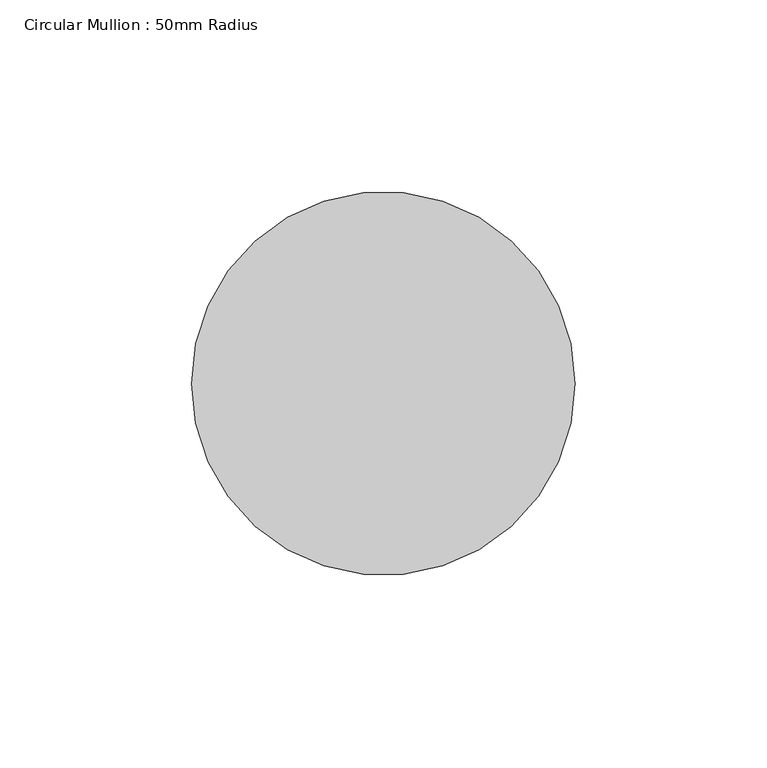
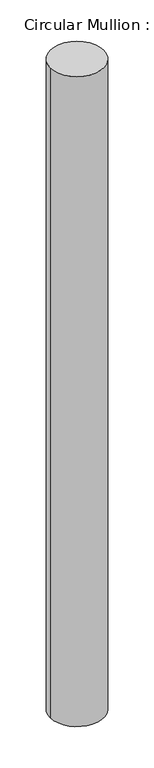
"""IFC4 building model written with IfcOpenShell, lengths in millimetres: member geometry, Circular Mullion : 50mm Radius."""

from ifc_helpers import new_model, si_unit, point, frame, origin, origin_2d, place, context, project, spatial, circle_curve, trimmed, segment, composite_curve, outline, extrude, source, transform, mapped, element, save


def circular_mullion_50mm_radius_a9a0c00b(model_context):
    return source(origin(), model_context, "Body", "SweptSolid", [
        extrude(outline(composite_curve([segment(trimmed(circle_curve(origin_2d(), 50.0), [point((50.0, 0.0))], [point((-50.0, 0.0))], False, "CARTESIAN"), True, "CONTINUOUS"), segment(trimmed(circle_curve(origin_2d(), 50.0), [point((-50.0, 0.0))], [point((50.0, 0.0))], False, "CARTESIAN"), True, "CONTINUOUS")], self_intersect=False)), frame((0.0, 0.0, -1287.9708847), z_axis=(0.0, 0.0, 1.0), x_axis=(1.0, 0.0, 0.0)), (0.0, 0.0, 1.0), 1287.9708847),
    ])


if __name__ == "__main__":
    model = new_model("IFC4")
    model_context = context("Model", 3, world=origin())
    ifc_project = project(units=[si_unit("LENGTHUNIT", "METRE", prefix="MILLI")], contexts=[model_context])
    site = spatial("IfcSite", under=ifc_project)
    building = spatial("IfcBuilding", under=site)
    placement = place(None, origin())
    circular_mullion_50mm_radius_shape = circular_mullion_50mm_radius_a9a0c00b(model_context)
    element("IfcMember", 1, ObjectType="Circular Mullion : 50mm Radius", at=placement, inside=building, context=model_context, shape_type="MappedRepresentation", body=[
        mapped(circular_mullion_50mm_radius_shape, transform((0.0, 0.0, 0.0), x_axis=(1.0, 0.0, 0.0), y_axis=(0.0, 1.0, 0.0), z_axis=(0.0, 0.0, 1.0))),
    ])
    save(model, "model.ifc")

# Revit data of these elements
# Type "Circular Mullion : 50mm Radius"
#   built-in parameter 1007350 = 0.164042 (stored number, unit not read)
# Element 1 (IfcMember, "Circular Mullion : 50mm Radius")
#   Materials on its faces: "Aluminium"
# Materials
#   "Aluminium": class "Metal", colour RGB 247 247 247, transparency 0, Description = "Aluminium 6061", Cost = 0
